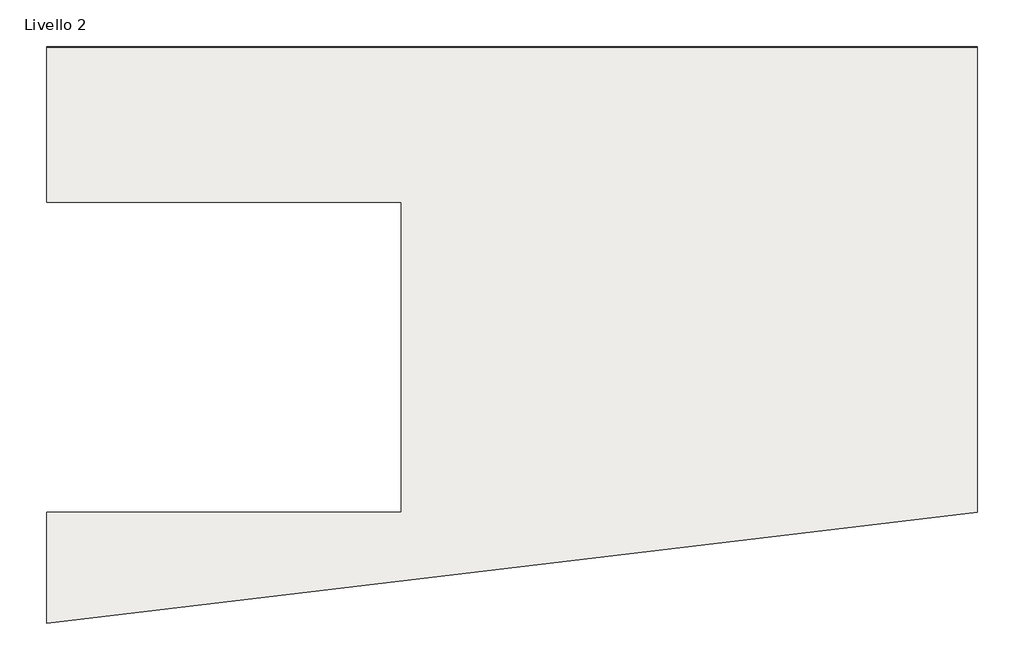
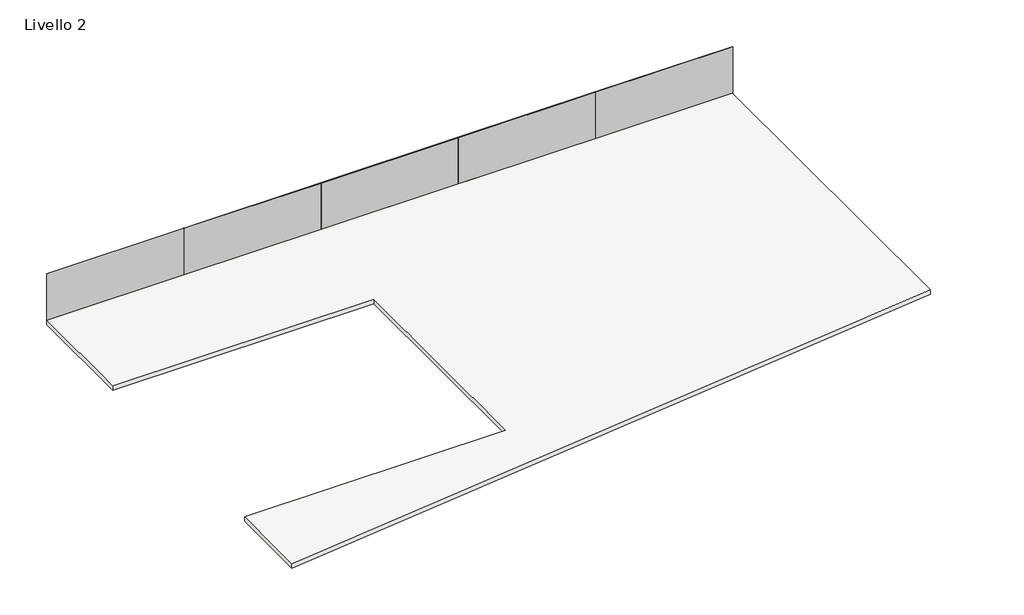
# One storey: 5 plates, 1 slab.
"""IFC4 building model written with IfcOpenShell, lengths in millimetres."""

import ifcopenshell
import ifcopenshell.guid

model = None  # the IFC model being written
_history = None  # IfcOwnerHistory: only IFC2X3 demands one
_inside = {}  # id of a spatial element -> (the spatial element, [elements in it])
_under = {}  # id of a project, library or spatial element -> (it, [spatial elements below it])
_declared = {}  # id of a project -> (the project, [libraries it declares])
_typed = {}  # id of a type object -> (the type object, [elements of that type])
_made_of = {}  # id of a material, layer set ... -> (it, [elements and type objects made of it])


def new_model(schema):
    """Start an empty IFC model of exactly this schema.

    Asked for "IFC4X3", IfcOpenShell would pick the latest addendum, in which some entities
    have other attributes; the version numbers below select the first issue.
    IFC2X3 requires an IfcOwnerHistory on every rooted entity: one is made here for all.
    """
    global model, _history
    if schema == "IFC4X3":
        model = ifcopenshell.file(schema_version=(4, 3, 0, 0))
    else:
        model = ifcopenshell.file(schema=schema)
    _inside.clear()
    _under.clear()
    _declared.clear()
    _typed.clear()
    _made_of.clear()
    _history = None
    if model.schema == "IFC2X3":
        org = make("IfcOrganization", Name="unknown")
        user = make(
            "IfcPersonAndOrganization",
            ThePerson=make("IfcPerson", FamilyName="unknown"),
            TheOrganization=org,
        )
        app = make(
            "IfcApplication",
            ApplicationDeveloper=org,
            Version="unknown",
            ApplicationFullName="unknown",
            ApplicationIdentifier="unknown",
        )
        _history = make(
            "IfcOwnerHistory",
            OwningUser=user,
            OwningApplication=app,
            ChangeAction="ADDED",
            CreationDate=0,
        )
    return model


def make(cls, **values):
    """One entity of the class cls with the attributes given. An attribute that is None is left unset."""
    return model.create_entity(
        cls, **{name: value for name, value in values.items() if value is not None}
    )


def rooted(cls, **values):
    """An entity with a GlobalId (a new one), such as an element, a storey or a relation."""
    return make(cls, GlobalId=ifcopenshell.guid.new(), OwnerHistory=_history, **values)


def si_unit(unit_type, name, prefix=None):
    """IfcSIUnit, for example si_unit("LENGTHUNIT", "METRE", prefix="MILLI")."""
    return make("IfcSIUnit", UnitType=unit_type, Prefix=prefix, Name=name)


def assignment(units):
    """IfcUnitAssignment: the units of a project."""
    return None if units is None else make("IfcUnitAssignment", Units=units)


def point(xyz):
    """IfcCartesianPoint."""
    return None if xyz is None else make("IfcCartesianPoint", Coordinates=xyz)


def direction(xyz):
    """IfcDirection."""
    return None if xyz is None else make("IfcDirection", DirectionRatios=xyz)


def frame(location, z_axis=None, x_axis=None):
    """IfcAxis2Placement3D, a coordinate frame: its origin and axes. An axis left out is left unset."""
    return make(
        "IfcAxis2Placement3D",
        Location=point(location),
        Axis=direction(z_axis),
        RefDirection=direction(x_axis),
    )


def origin():
    """The frame at (0, 0, 0) with its axes left unset."""
    return frame((0.0, 0.0, 0.0))


def origin_with_axes():
    """The frame at (0, 0, 0) with the z axis (0, 0, 1) and the x axis (1, 0, 0) written out."""
    return frame((0.0, 0.0, 0.0), z_axis=(0.0, 0.0, 1.0), x_axis=(1.0, 0.0, 0.0))


def place(relative_to, where):
    """IfcLocalPlacement: puts the frame where relative to a parent placement (None: the world)."""
    return make(
        "IfcLocalPlacement", PlacementRelTo=relative_to, RelativePlacement=where
    )


def context(
    kind, dimensions, precision=None, world=None, true_north=None, identifier=None
):
    """IfcGeometricRepresentationContext, for example the 3D "Model" context."""
    return make(
        "IfcGeometricRepresentationContext",
        ContextIdentifier=identifier,
        ContextType=kind,
        CoordinateSpaceDimension=dimensions,
        Precision=precision,
        WorldCoordinateSystem=world,
        TrueNorth=true_north,
    )


def project(units=None, contexts=None):
    """IfcProject with its units and contexts."""
    return rooted(
        "IfcProject",
        Name="project",
        RepresentationContexts=contexts,
        UnitsInContext=assignment(units),
    )


def spatial(cls, under=None, at=None, **own):
    """A site, building, storey or space (cls), placed at a placement, below another one or the project."""
    s = rooted(cls, ObjectPlacement=at, **own)
    if under is not None:
        _under.setdefault(under.id(), (under, []))[1].append(s)
    return s


def polyline(points):
    """IfcPolyline through the points."""
    return make("IfcPolyline", Points=[point(p) for p in points])


def outline(outer, holes=None, kind="AREA"):
    """IfcArbitraryClosedProfileDef: a profile drawn as a closed curve; with holes, ...WithVoids."""
    if holes is None:
        return make("IfcArbitraryClosedProfileDef", ProfileType=kind, OuterCurve=outer)
    return make(
        "IfcArbitraryProfileDefWithVoids",
        ProfileType=kind,
        OuterCurve=outer,
        InnerCurves=holes,
    )


def extrude(swept, where, along, depth):
    """IfcExtrudedAreaSolid: the profile swept, set in the frame where, extruded along a direction by depth."""
    return make(
        "IfcExtrudedAreaSolid",
        SweptArea=swept,
        Position=where,
        ExtrudedDirection=direction(along),
        Depth=depth,
    )


def shape(context_of_items, identifier, shape_type, items):
    """IfcShapeRepresentation: the items that make up one representation, for example the "Body"."""
    return make(
        "IfcShapeRepresentation",
        ContextOfItems=context_of_items,
        RepresentationIdentifier=identifier,
        RepresentationType=shape_type,
        Items=items,
    )


def source(mapping_origin, context_of_items, identifier, shape_type, items):
    """IfcRepresentationMap: a shape defined once, which mapped items show again and again."""
    return make(
        "IfcRepresentationMap",
        MappingOrigin=mapping_origin,
        MappedRepresentation=shape(context_of_items, identifier, shape_type, items),
    )


def transform(
    local_origin,
    x_axis=None,
    y_axis=None,
    z_axis=None,
    scale=None,
    scale2=None,
    scale3=None,
    uniform=True,
):
    """IfcCartesianTransformationOperator3D, or its non-uniform kind. x_axis, y_axis, z_axis: its Axis1, 2, 3."""
    if uniform:
        return make(
            "IfcCartesianTransformationOperator3D",
            Axis1=direction(x_axis),
            Axis2=direction(y_axis),
            LocalOrigin=point(local_origin),
            Scale=scale,
            Axis3=direction(z_axis),
        )
    return make(
        "IfcCartesianTransformationOperator3DnonUniform",
        Axis1=direction(x_axis),
        Axis2=direction(y_axis),
        LocalOrigin=point(local_origin),
        Scale=scale,
        Axis3=direction(z_axis),
        Scale2=scale2,
        Scale3=scale3,
    )


def mapped(mapping_source, mapping_target):
    """IfcMappedItem: shows the shape of a source again, moved by a transform."""
    return make(
        "IfcMappedItem", MappingSource=mapping_source, MappingTarget=mapping_target
    )


def made_of(thing, what):
    """Note that an element or type object is made of a material, layer set ...; save() writes the relation."""
    if what is not None:
        _made_of.setdefault(what.id(), (what, []))[1].append(thing)
    return thing


def element(
    cls,
    number,
    at=None,
    inside=None,
    cuts=None,
    type_object=None,
    material=None,
    context=None,
    identifier="Body",
    shape_type=None,
    held_by="IfcProductDefinitionShape",
    body=None,
    shapes=None,
    **own,
):
    """One element of the class cls, such as IfcWall. Its Tag is "e" and its number.

    at: its placement. inside: the storey or other place that contains it. cuts: it is an
    opening in that element (IfcRelVoidsElement). A single representation is given by context,
    identifier, shape_type and body (its items); several are given by shapes. held_by: the class
    of the entity that holds the representations. save() writes the other relations.
    """
    e = rooted(cls, Tag="e%d" % number, ObjectPlacement=at, **own)
    if body is not None:
        shapes = [shape(context, identifier, shape_type, body)]
    if shapes is not None:
        e.Representation = make(held_by, Representations=shapes)
    if inside is not None:
        _inside.setdefault(inside.id(), (inside, []))[1].append(e)
    if cuts is not None:
        rooted(
            "IfcRelVoidsElement", RelatingBuildingElement=cuts, RelatedOpeningElement=e
        )
    if type_object is not None:
        _typed.setdefault(type_object.id(), (type_object, []))[1].append(e)
    return made_of(e, material)


def aggregate(whole, parts):
    """IfcRelAggregates: a whole, such as a stair, and the parts it consists of."""
    return rooted("IfcRelAggregates", RelatingObject=whole, RelatedObjects=parts)


def save(model, path):
    """Write the relations noted so far, then the file.

    IfcRelAggregates (storeys below a building ...), IfcRelContainedInSpatialStructure (elements
    in a storey), IfcRelDefinesByType, IfcRelAssociatesMaterial and IfcRelDeclares: one each for
    every whole, place, type object, material and project.
    """
    for whole, parts in _under.values():
        aggregate(whole, parts)
    for where, things in _inside.values():
        rooted(
            "IfcRelContainedInSpatialStructure",
            RelatedElements=things,
            RelatingStructure=where,
        )
    for kind, things in _typed.values():
        rooted("IfcRelDefinesByType", RelatedObjects=things, RelatingType=kind)
    for what, things in _made_of.values():
        rooted("IfcRelAssociatesMaterial", RelatedObjects=things, RelatingMaterial=what)
    for by, libraries in _declared.values():
        rooted("IfcRelDeclares", RelatingContext=by, RelatedDefinitions=libraries)
    model.write(path)


def pannello_sistema_vetrato_29ff3466(model_context):
    return source(origin(), model_context, "Body", "SweptSolid", [
        extrude(outline(polyline([(4200.0000001, -15.0), (-4200.0000001, -15.0), (-4200.0000001, 15.0), (4200.0000001, 15.0), (4200.0000001, -15.0)])), origin_with_axes(), (0.0, 0.0, 1.0), 3000.0),
    ])


model = new_model("IFC4")

# Units and contexts
model_context = context("Model", 3, world=origin())
ifc_project = project(units=[si_unit("LENGTHUNIT", "METRE", prefix="MILLI")], contexts=[model_context])

# Site, building, storey
site = spatial("IfcSite", under=ifc_project)
building = spatial("IfcBuilding", under=site)
storey = spatial("IfcBuildingStorey", under=building, Name="Livello 2", Elevation=6000.0)

# Plates
placement = place(None, origin())
pannello_sistema_vetrato_shape = pannello_sistema_vetrato_29ff3466(model_context)
element("IfcPlate", 1, ObjectType="Pannello sistema : Vetrato", at=placement, inside=storey, context=model_context, shape_type="MappedRepresentation", body=[
    mapped(pannello_sistema_vetrato_shape, transform((-20934.9893485, 13197.4454735, 6000.0), x_axis=(1.0, 0.0, 0.0), y_axis=(0.0, 1.0, 0.0), z_axis=(0.0, 0.0, 1.0))),
])
element("IfcPlate", 2, ObjectType="Pannello sistema : Vetrato", at=placement, inside=storey, context=model_context, shape_type="MappedRepresentation", body=[
    mapped(pannello_sistema_vetrato_shape, transform((-12534.9893485, 13197.4454735, 6000.0), x_axis=(1.0, 0.0, 0.0), y_axis=(0.0, 1.0, 0.0), z_axis=(0.0, 0.0, 1.0))),
])
element("IfcPlate", 3, ObjectType="Pannello sistema : Vetrato", at=placement, inside=storey, context=model_context, shape_type="MappedRepresentation", body=[
    mapped(pannello_sistema_vetrato_shape, transform((-4134.9893486, 13197.4454735, 6000.0), x_axis=(1.0, 0.0, 0.0), y_axis=(0.0, 1.0, 0.0), z_axis=(0.0, 0.0, 1.0))),
])
element("IfcPlate", 4, ObjectType="Pannello sistema : Vetrato", at=placement, inside=storey, context=model_context, shape_type="MappedRepresentation", body=[
    mapped(pannello_sistema_vetrato_shape, transform((4265.0106513, 13197.4454735, 6000.0), x_axis=(1.0, 0.0, 0.0), y_axis=(0.0, 1.0, 0.0), z_axis=(0.0, 0.0, 1.0))),
])
element("IfcPlate", 5, ObjectType="Pannello sistema : Vetrato", at=placement, inside=storey, context=model_context, shape_type="MappedRepresentation", body=[
    mapped(pannello_sistema_vetrato_shape, transform((12665.0106513, 13197.4454735, 6000.0), x_axis=(1.0, 0.0, 0.0), y_axis=(0.0, 1.0, 0.0), z_axis=(0.0, 0.0, 1.0))),
])

# Slab
element("IfcSlab", 6, ObjectType="Latero Cementizio - 30 cm", at=placement, inside=storey, context=model_context, shape_type="SweptSolid", body=[
    extrude(outline(polyline([(-25134.9893486, -7802.5545265), (-9134.9893486, -7802.5545265), (-9134.9893486, 6197.4454735), (-25134.9893486, 6197.4454735), (-25134.9893486, 13197.4454735), (16865.0106514, 13197.4454735), (16865.0106514, -7802.5545265), (-25134.9893486, -12802.5545265), (-25134.9893486, -7802.5545265)])), frame((0.0, 0.0, 5700.0), z_axis=(0.0, 0.0, 1.0), x_axis=(1.0, 0.0, 0.0)), (0.0, 0.0, 1.0), 300.0),
])

save(model, "model.ifc")

# Revit data of these elements
# Type "Pannello sistema : Vetrato"
#   Construction Type Id = "GSP4R"
#   Analytic Construction = "Vetrata singola Pilkington 1/8 in"
#   Visual Light Transmittance = 0.9
#   Solar Heat Gain Coefficient = 0.86
#   Heat Transfer Coefficient (U) = 6.7069 W/(m²·K)
# Type "Latero Cementizio - 30 cm"
#   Keynote = "S/3"
#   Function = 0
#   Layers, outside or top first: 0.02 m "Ceramica bianca" (function 4); 0.065 m "Sabbia e Calcestruzzo" (function 2); 0.04 m "Calcestruzzo" (function 1); 0.16 m "Laterizio (2)" (function 1); 0.015 m "Intonaco - Bianco" (function 5)
# Elements 1, 2, 3, 4, 5 (IfcPlate, "Pannello sistema : Vetrato")
#   Phase Created = Stato di Progetto
#   Materials on its faces: "Default - Vetro"
# Element 6 (IfcSlab, "Latero Cementizio - 30 cm")
#   built-in parameter 1001955 = 1.5708 (stored number, unit not read)
#   Height Offset From Level = 0.00 m
#   Phase Created = Stato di Progetto
#   Materials on its faces: "Intonaco - Bianco", "Ceramica bianca"
# Materials
#   "Ceramica bianca": class "Ceramica", colour RGB 210 210 210, transparency 0, Description = "Finitura interna - Piastrelle di ceramica incollate", Cost = 0
#   "Sabbia e Calcestruzzo": class "Calcestruzzo", colour RGB 127 127 127, transparency 0, Description = "Magrone - Sabbia e cemento", Cost = 0
#   "Calcestruzzo": class "Calcestruzzo", colour RGB 192 192 192, transparency 0, Description = "Calcestruzzo - Cemento Portland", Cost = 0
#   "Laterizio (2)": class "Mattone", colour RGB 255 128 64, transparency 0, Description = "Pignatta h 16 cm", Cost = 0
#   "Intonaco - Bianco": class "Intonaco", colour RGB 249 249 249, transparency 0, Description = "Verniciatura", Cost = 0
#   "Default - Vetro": class "Vetro", colour RGB 208 208 208, transparency 0.7, Cost = 0
